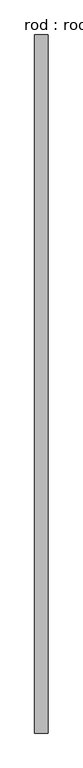
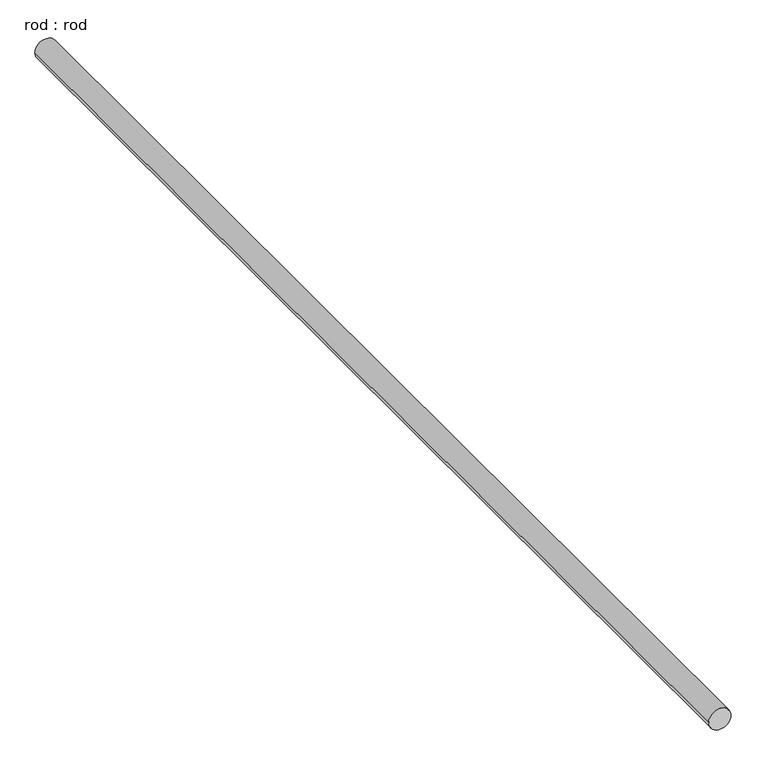
"""IFC4 building model written with IfcOpenShell, lengths in millimetres: proxy geometry, rod : rod."""

from ifc_helpers import new_model, si_unit, point, frame, frame_2d, origin, place, context, project, spatial, circle_curve, trimmed, segment, composite_curve, outline, extrude, source, transform, mapped, element, save


def rod_rod_f173f8bf(model_context):
    return source(origin(), model_context, "Body", "SweptSolid", [
        extrude(outline(composite_curve([segment(trimmed(circle_curve(frame_2d((0.0108462, 0.0)), 200.0), [point((0.0108462, 200.0))], [point((0.0108462, -200.0))], False, "CARTESIAN"), True, "CONTINUOUS"), segment(trimmed(circle_curve(frame_2d((0.0108462, 0.0)), 200.0), [point((0.0108462, -200.0))], [point((0.0108462, 200.0))], False, "CARTESIAN"), True, "CONTINUOUS")], self_intersect=False)), frame((0.0, -6424.3594144, 0.0), z_axis=(0.0, 1.0, 0.0), x_axis=(0.0, 0.0, 1.0)), (0.0, 0.0, 1.0), 21034.1760595),
    ])


if __name__ == "__main__":
    model = new_model("IFC4")
    model_context = context("Model", 3, world=origin())
    ifc_project = project(units=[si_unit("LENGTHUNIT", "METRE", prefix="MILLI")], contexts=[model_context])
    site = spatial("IfcSite", under=ifc_project)
    building = spatial("IfcBuilding", under=site)
    placement = place(None, origin())
    rod_rod_shape = rod_rod_f173f8bf(model_context)
    element("IfcBuildingElementProxy", 1, Name="rod : rod", ObjectType="rod : rod", at=placement, inside=building, context=model_context, shape_type="MappedRepresentation", body=[
        mapped(rod_rod_shape, transform((0.0, 0.0, 0.0), x_axis=(1.0, 0.0, 0.0), y_axis=(0.0, 1.0, 0.0), z_axis=(0.0, 0.0, 1.0))),
    ])
    save(model, "model.ifc")

# Revit data of these elements
# Type "rod : rod"
#   Default Elevation = 0
